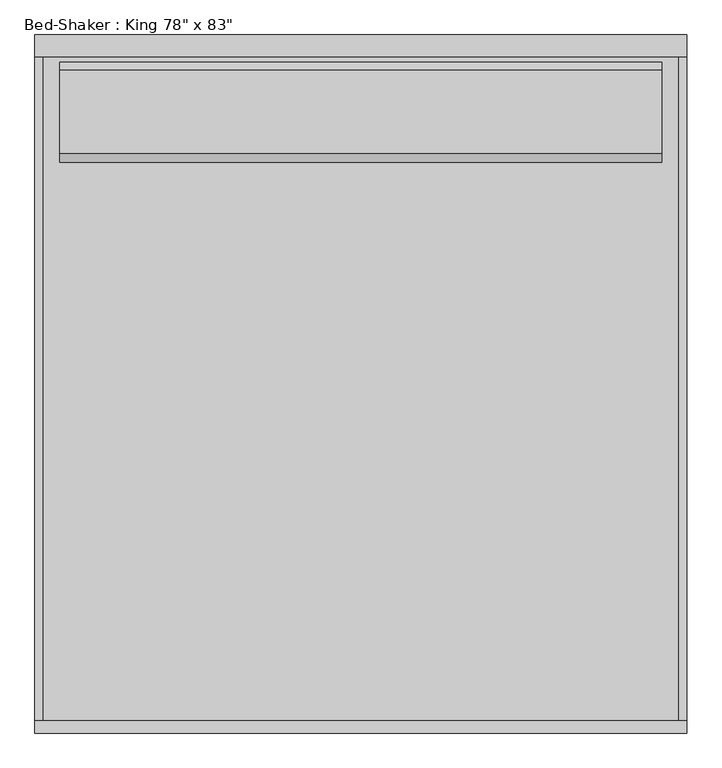
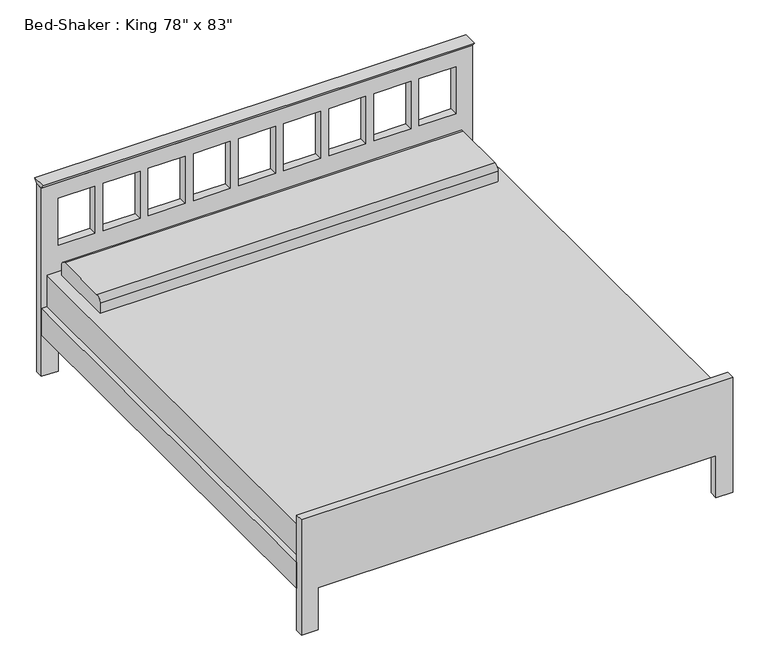
"""IFC4 building model written with IfcOpenShell, lengths in millimetres: furniture geometry."""

import ifcopenshell
import ifcopenshell.guid

model = None  # the IFC model being written
_history = None  # IfcOwnerHistory: only IFC2X3 demands one
_inside = {}  # id of a spatial element -> (the spatial element, [elements in it])
_under = {}  # id of a project, library or spatial element -> (it, [spatial elements below it])
_declared = {}  # id of a project -> (the project, [libraries it declares])
_typed = {}  # id of a type object -> (the type object, [elements of that type])
_made_of = {}  # id of a material, layer set ... -> (it, [elements and type objects made of it])


def new_model(schema):
    """Start an empty IFC model of exactly this schema.

    Asked for "IFC4X3", IfcOpenShell would pick the latest addendum, in which some entities
    have other attributes; the version numbers below select the first issue.
    IFC2X3 requires an IfcOwnerHistory on every rooted entity: one is made here for all.
    """
    global model, _history
    if schema == "IFC4X3":
        model = ifcopenshell.file(schema_version=(4, 3, 0, 0))
    else:
        model = ifcopenshell.file(schema=schema)
    _inside.clear()
    _under.clear()
    _declared.clear()
    _typed.clear()
    _made_of.clear()
    _history = None
    if model.schema == "IFC2X3":
        org = make("IfcOrganization", Name="unknown")
        user = make(
            "IfcPersonAndOrganization",
            ThePerson=make("IfcPerson", FamilyName="unknown"),
            TheOrganization=org,
        )
        app = make(
            "IfcApplication",
            ApplicationDeveloper=org,
            Version="unknown",
            ApplicationFullName="unknown",
            ApplicationIdentifier="unknown",
        )
        _history = make(
            "IfcOwnerHistory",
            OwningUser=user,
            OwningApplication=app,
            ChangeAction="ADDED",
            CreationDate=0,
        )
    return model


def make(cls, **values):
    """One entity of the class cls with the attributes given. An attribute that is None is left unset."""
    return model.create_entity(
        cls, **{name: value for name, value in values.items() if value is not None}
    )


def rooted(cls, **values):
    """An entity with a GlobalId (a new one), such as an element, a storey or a relation."""
    return make(cls, GlobalId=ifcopenshell.guid.new(), OwnerHistory=_history, **values)


def si_unit(unit_type, name, prefix=None):
    """IfcSIUnit, for example si_unit("LENGTHUNIT", "METRE", prefix="MILLI")."""
    return make("IfcSIUnit", UnitType=unit_type, Prefix=prefix, Name=name)


def assignment(units):
    """IfcUnitAssignment: the units of a project."""
    return None if units is None else make("IfcUnitAssignment", Units=units)


def point(xyz):
    """IfcCartesianPoint."""
    return None if xyz is None else make("IfcCartesianPoint", Coordinates=xyz)


def direction(xyz):
    """IfcDirection."""
    return None if xyz is None else make("IfcDirection", DirectionRatios=xyz)


def frame(location, z_axis=None, x_axis=None):
    """IfcAxis2Placement3D, a coordinate frame: its origin and axes. An axis left out is left unset."""
    return make(
        "IfcAxis2Placement3D",
        Location=point(location),
        Axis=direction(z_axis),
        RefDirection=direction(x_axis),
    )


def frame_2d(location, x_axis=None):
    """IfcAxis2Placement2D, a coordinate frame in the plane: its origin and x axis."""
    return make(
        "IfcAxis2Placement2D", Location=point(location), RefDirection=direction(x_axis)
    )


def origin():
    """The frame at (0, 0, 0) with its axes left unset."""
    return frame((0.0, 0.0, 0.0))


def place(relative_to, where):
    """IfcLocalPlacement: puts the frame where relative to a parent placement (None: the world)."""
    return make(
        "IfcLocalPlacement", PlacementRelTo=relative_to, RelativePlacement=where
    )


def context(
    kind, dimensions, precision=None, world=None, true_north=None, identifier=None
):
    """IfcGeometricRepresentationContext, for example the 3D "Model" context."""
    return make(
        "IfcGeometricRepresentationContext",
        ContextIdentifier=identifier,
        ContextType=kind,
        CoordinateSpaceDimension=dimensions,
        Precision=precision,
        WorldCoordinateSystem=world,
        TrueNorth=true_north,
    )


def project(units=None, contexts=None):
    """IfcProject with its units and contexts."""
    return rooted(
        "IfcProject",
        Name="project",
        RepresentationContexts=contexts,
        UnitsInContext=assignment(units),
    )


def spatial(cls, under=None, at=None, **own):
    """A site, building, storey or space (cls), placed at a placement, below another one or the project."""
    s = rooted(cls, ObjectPlacement=at, **own)
    if under is not None:
        _under.setdefault(under.id(), (under, []))[1].append(s)
    return s


def polyline(points):
    """IfcPolyline through the points."""
    return make("IfcPolyline", Points=[point(p) for p in points])


def circle_curve(where, radius):
    """IfcCircle in the frame where."""
    return make("IfcCircle", Position=where, Radius=radius)


def trimmed(basis, trim1, trim2, sense, master):
    """IfcTrimmedCurve: the piece of a basis curve between two trims."""
    return make(
        "IfcTrimmedCurve",
        BasisCurve=basis,
        Trim1=trim1,
        Trim2=trim2,
        SenseAgreement=sense,
        MasterRepresentation=master,
    )


def segment(curve, same_sense, transition):
    """IfcCompositeCurveSegment."""
    return make(
        "IfcCompositeCurveSegment",
        Transition=transition,
        SameSense=same_sense,
        ParentCurve=curve,
    )


def composite_curve(segments, self_intersect=None):
    """IfcCompositeCurve: segments joined end to end."""
    return make("IfcCompositeCurve", Segments=segments, SelfIntersect=self_intersect)


def outline(outer, holes=None, kind="AREA"):
    """IfcArbitraryClosedProfileDef: a profile drawn as a closed curve; with holes, ...WithVoids."""
    if holes is None:
        return make("IfcArbitraryClosedProfileDef", ProfileType=kind, OuterCurve=outer)
    return make(
        "IfcArbitraryProfileDefWithVoids",
        ProfileType=kind,
        OuterCurve=outer,
        InnerCurves=holes,
    )


def extrude(swept, where, along, depth):
    """IfcExtrudedAreaSolid: the profile swept, set in the frame where, extruded along a direction by depth."""
    return make(
        "IfcExtrudedAreaSolid",
        SweptArea=swept,
        Position=where,
        ExtrudedDirection=direction(along),
        Depth=depth,
    )


def shape(context_of_items, identifier, shape_type, items):
    """IfcShapeRepresentation: the items that make up one representation, for example the "Body"."""
    return make(
        "IfcShapeRepresentation",
        ContextOfItems=context_of_items,
        RepresentationIdentifier=identifier,
        RepresentationType=shape_type,
        Items=items,
    )


def source(mapping_origin, context_of_items, identifier, shape_type, items):
    """IfcRepresentationMap: a shape defined once, which mapped items show again and again."""
    return make(
        "IfcRepresentationMap",
        MappingOrigin=mapping_origin,
        MappedRepresentation=shape(context_of_items, identifier, shape_type, items),
    )


def transform(
    local_origin,
    x_axis=None,
    y_axis=None,
    z_axis=None,
    scale=None,
    scale2=None,
    scale3=None,
    uniform=True,
):
    """IfcCartesianTransformationOperator3D, or its non-uniform kind. x_axis, y_axis, z_axis: its Axis1, 2, 3."""
    if uniform:
        return make(
            "IfcCartesianTransformationOperator3D",
            Axis1=direction(x_axis),
            Axis2=direction(y_axis),
            LocalOrigin=point(local_origin),
            Scale=scale,
            Axis3=direction(z_axis),
        )
    return make(
        "IfcCartesianTransformationOperator3DnonUniform",
        Axis1=direction(x_axis),
        Axis2=direction(y_axis),
        LocalOrigin=point(local_origin),
        Scale=scale,
        Axis3=direction(z_axis),
        Scale2=scale2,
        Scale3=scale3,
    )


def mapped(mapping_source, mapping_target):
    """IfcMappedItem: shows the shape of a source again, moved by a transform."""
    return make(
        "IfcMappedItem", MappingSource=mapping_source, MappingTarget=mapping_target
    )


def made_of(thing, what):
    """Note that an element or type object is made of a material, layer set ...; save() writes the relation."""
    if what is not None:
        _made_of.setdefault(what.id(), (what, []))[1].append(thing)
    return thing


def element(
    cls,
    number,
    at=None,
    inside=None,
    cuts=None,
    type_object=None,
    material=None,
    context=None,
    identifier="Body",
    shape_type=None,
    held_by="IfcProductDefinitionShape",
    body=None,
    shapes=None,
    **own,
):
    """One element of the class cls, such as IfcWall. Its Tag is "e" and its number.

    at: its placement. inside: the storey or other place that contains it. cuts: it is an
    opening in that element (IfcRelVoidsElement). A single representation is given by context,
    identifier, shape_type and body (its items); several are given by shapes. held_by: the class
    of the entity that holds the representations. save() writes the other relations.
    """
    e = rooted(cls, Tag="e%d" % number, ObjectPlacement=at, **own)
    if body is not None:
        shapes = [shape(context, identifier, shape_type, body)]
    if shapes is not None:
        e.Representation = make(held_by, Representations=shapes)
    if inside is not None:
        _inside.setdefault(inside.id(), (inside, []))[1].append(e)
    if cuts is not None:
        rooted(
            "IfcRelVoidsElement", RelatingBuildingElement=cuts, RelatedOpeningElement=e
        )
    if type_object is not None:
        _typed.setdefault(type_object.id(), (type_object, []))[1].append(e)
    return made_of(e, material)


def aggregate(whole, parts):
    """IfcRelAggregates: a whole, such as a stair, and the parts it consists of."""
    return rooted("IfcRelAggregates", RelatingObject=whole, RelatedObjects=parts)


def save(model, path):
    """Write the relations noted so far, then the file.

    IfcRelAggregates (storeys below a building ...), IfcRelContainedInSpatialStructure (elements
    in a storey), IfcRelDefinesByType, IfcRelAssociatesMaterial and IfcRelDeclares: one each for
    every whole, place, type object, material and project.
    """
    for whole, parts in _under.values():
        aggregate(whole, parts)
    for where, things in _inside.values():
        rooted(
            "IfcRelContainedInSpatialStructure",
            RelatedElements=things,
            RelatingStructure=where,
        )
    for kind, things in _typed.values():
        rooted("IfcRelDefinesByType", RelatedObjects=things, RelatingType=kind)
    for what, things in _made_of.values():
        rooted("IfcRelAssociatesMaterial", RelatedObjects=things, RelatingMaterial=what)
    for by, libraries in _declared.values():
        rooted("IfcRelDeclares", RelatingContext=by, RelatedDefinitions=libraries)
    model.write(path)


def furniture_29cd36cd(model_context):
    return source(origin(), model_context, "Body", "SweptSolid", [
        extrude(outline(polyline([(-38.1, 914.4), (-51.9545455, 933.45), (13.8545455, 933.45), (0.0, 914.4), (-38.1, 914.4)])), frame((-1009.4365546, 0.0, 0.0), z_axis=(1.0, 0.0, 0.0), x_axis=(0.0, 1.0, 0.0)), (0.0, 0.0, 1.0), 1981.2533613),
        extrude(outline(composite_curve([segment(polyline([(-373.2486637, 482.6), (-373.2486637, 533.4)]), True, "CONTINUOUS"), segment(trimmed(circle_curve(frame_2d((-347.8486637, 533.4)), 25.4), [point((-373.2486637, 533.4))], [point((-347.8486637, 558.8))], False, "CARTESIAN"), True, "CONTINUOUS"), segment(polyline([(-347.8486637, 558.8), (-93.8486637, 558.8)]), True, "CONTINUOUS"), segment(trimmed(circle_curve(frame_2d((-93.8486637, 533.4)), 25.4), [point((-93.8486637, 558.8))], [point((-68.4486637, 533.4))], False, "CARTESIAN"), True, "CONTINUOUS"), segment(polyline([(-68.4486637, 533.4), (-68.4486637, 482.6), (-373.2486637, 482.6)]), True, "CONTINUOUS")], self_intersect=False)), frame((-933.45, 0.0, 0.0), z_axis=(1.0, 0.0, 0.0), x_axis=(0.0, 1.0, 0.0)), (0.0, 0.0, 1.0), 1828.8),
        extrude(outline(polyline([(946.15, -38.1), (946.15, -2070.1), (-984.25, -2070.1), (-984.25, -38.1), (946.15, -38.1)])), frame((0.0, 0.0, 228.6), z_axis=(0.0, 0.0, 1.0), x_axis=(1.0, 0.0, 0.0)), (0.0, 0.0, 1.0), 254.0),
        extrude(outline(polyline([(946.15, -2070.1), (946.15, -38.1), (971.55, -38.1), (971.55, -2070.1), (946.15, -2070.1)])), frame((0.0, 0.0, 203.0994861), z_axis=(0.0, 0.0, 1.0), x_axis=(1.0, 0.0, 0.0)), (0.0, 0.0, 1.0), 127.0),
        extrude(outline(polyline([(-1009.65, -2070.1), (-1009.65, -38.1), (-984.25, -38.1), (-984.25, -2070.1), (-1009.65, -2070.1)])), frame((0.0, 0.0, 203.5755296), z_axis=(0.0, 0.0, 1.0), x_axis=(1.0, 0.0, 0.0)), (0.0, 0.0, 1.0), 127.0),
        extrude(outline(polyline([(0.0, -933.45), (203.2, -933.45), (203.2, 895.35), (0.0, 895.35), (0.0, 971.55), (558.8, 971.55), (558.8, -1009.65), (0.0, -1009.65), (0.0, -933.45)])), frame((0.0, -2108.2, 0.0), z_axis=(0.0, 1.0, 0.0), x_axis=(0.0, 0.0, 1.0)), (0.0, 0.0, 1.0), 38.1),
        extrude(outline(polyline([(914.4, 971.8168067), (914.4, -1009.4365546), (0.0, -1009.4365546), (0.0, -933.45), (203.2, -933.45), (203.2, 895.35), (0.0, 895.35), (0.0, 971.8168067), (914.4, 971.8168067)]), holes=[polyline([(838.2, -764.1166667), (609.6, -764.1166667), (609.6, -933.45), (838.2, -933.45), (838.2, -764.1166667)]), polyline([(838.2, -556.6833333), (609.6, -556.6833333), (609.6, -726.0166667), (838.2, -726.0166667), (838.2, -556.6833333)]), polyline([(838.2, -349.25), (609.6, -349.25), (609.6, -518.5833333), (838.2, -518.5833333), (838.2, -349.25)]), polyline([(838.2, -141.8166667), (609.6, -141.8166667), (609.6, -311.15), (838.2, -311.15), (838.2, -141.8166667)]), polyline([(838.2, 273.05), (609.6, 273.05), (609.6, 103.7166667), (838.2, 103.7166667), (838.2, 273.05)]), polyline([(838.2, 480.4833333), (609.6, 480.4833333), (609.6, 311.15), (838.2, 311.15), (838.2, 480.4833333)]), polyline([(838.2, 687.9166667), (609.6, 687.9166667), (609.6, 518.5833333), (838.2, 518.5833333), (838.2, 687.9166667)]), polyline([(838.2, 895.35), (609.6, 895.35), (609.6, 726.0166667), (838.2, 726.0166667), (838.2, 895.35)]), polyline([(838.2, 65.6166667), (609.6, 65.6166667), (609.6, -103.7166667), (838.2, -103.7166667), (838.2, 65.6166667)])]), frame((0.0, -38.1, 0.0), z_axis=(0.0, 1.0, 0.0), x_axis=(0.0, 0.0, 1.0)), (0.0, 0.0, 1.0), 38.1),
    ])


if __name__ == "__main__":
    model = new_model("IFC4")
    model_context = context("Model", 3, world=origin())
    ifc_project = project(units=[si_unit("LENGTHUNIT", "METRE", prefix="MILLI")], contexts=[model_context])
    site = spatial("IfcSite", under=ifc_project)
    building = spatial("IfcBuilding", under=site)
    placement = place(None, origin())
    furniture_shape = furniture_29cd36cd(model_context)
    element("IfcFurniture", 1, ObjectType="Bed-Shaker : King 78\" x 83\"", at=placement, inside=building, context=model_context, shape_type="MappedRepresentation", body=[
        mapped(furniture_shape, transform((0.0, 0.0, 0.0), x_axis=(1.0, 0.0, 0.0), y_axis=(0.0, 1.0, 0.0), z_axis=(0.0, 0.0, 1.0))),
    ])
    save(model, "model.ifc")

# Revit data of these elements
# Project information
#   Project Issue Date = "Issue Date"
#   Project Status = "Project Status"
#   Client Name = "Owner"
#   Project Address = "Enter address here"
#   Project Name = "Project Name"
#   Project Number = "Project Number"
# Type "Bed-Shaker : King 78\" x 83\""
#   Assembly Code = "E2020200"
#   Length = 6' - 11"
#   Width = 6' - 6"
#   Frame Material = Birch
#   Mattress Material = Linen, White
# Element 1 (IfcFurniture, "Bed-Shaker : King 78\" x 83\"")
#   Materials on its faces: "Birch", "Linen, White"
# Materials
#   "Birch": class "Wood", colour RGB 224 178 126, transparency 0, Description = "Betula Alleghaniensis", Cost = 0
#   "Linen, White": class "Textile", colour RGB 247 247 239, transparency 0, Description = "Linen, white", Cost = 0
